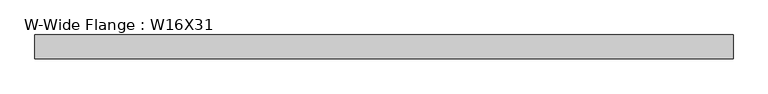
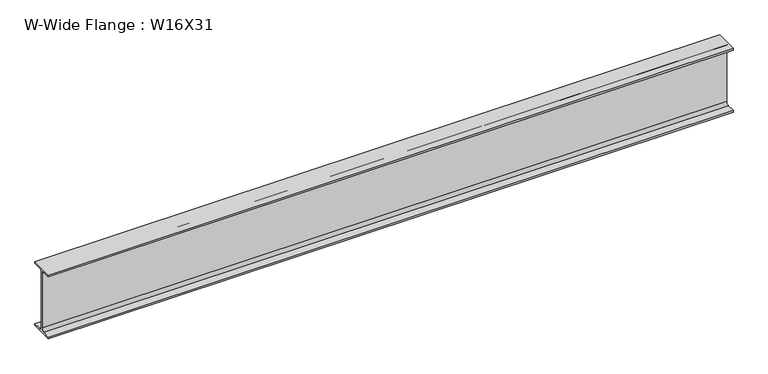
"""IFC4 building model written with IfcOpenShell, lengths in millimetres: beam geometry, W-Wide Flange : W16X31."""

from ifc_helpers import new_model, si_unit, point, frame, frame_2d, origin, place, context, project, spatial, polyline, circle_curve, trimmed, segment, composite_curve, outline, extrude, source, transform, mapped, element, save


def w_wide_flange_w16x31_034e3d4c(model_context):
    return source(origin(), model_context, "Body", "SweptSolid", [
        extrude(outline(composite_curve([segment(polyline([(70.231, -190.754), (70.231, -201.93), (-70.231, -201.93), (-70.231, -190.754), (-20.8915, -190.754)]), True, "CONTINUOUS"), segment(trimmed(circle_curve(frame_2d((-20.8915, -173.355)), 17.399), [point((-20.8915, -190.754))], [point((-3.4925, -173.355))], True, "CARTESIAN"), True, "CONTINUOUS"), segment(polyline([(-3.4925, -173.355), (-3.4925, 173.355)]), True, "CONTINUOUS"), segment(trimmed(circle_curve(frame_2d((-20.8915, 173.355)), 17.399), [point((-3.4925, 173.355))], [point((-20.8915, 190.754))], True, "CARTESIAN"), True, "CONTINUOUS"), segment(polyline([(-20.8915, 190.754), (-70.231, 190.754), (-70.231, 201.93), (70.231, 201.93), (70.231, 190.754), (20.8915, 190.754)]), True, "CONTINUOUS"), segment(trimmed(circle_curve(frame_2d((20.8915, 173.355)), 17.399), [point((20.8915, 190.754))], [point((3.4925, 173.355))], True, "CARTESIAN"), True, "CONTINUOUS"), segment(polyline([(3.4925, 173.355), (3.4925, -173.355)]), True, "CONTINUOUS"), segment(trimmed(circle_curve(frame_2d((20.8915, -173.355)), 17.399), [point((3.4925, -173.355))], [point((20.8915, -190.754))], True, "CARTESIAN"), True, "CONTINUOUS"), segment(polyline([(20.8915, -190.754), (70.231, -190.754)]), True, "CONTINUOUS")], self_intersect=False)), frame((-2052.124346, 0.0, 0.0), z_axis=(1.0, 0.0, 0.0), x_axis=(0.0, 1.0, 0.0)), (0.0, 0.0, 1.0), 4104.248692),
    ])


if __name__ == "__main__":
    model = new_model("IFC4")
    model_context = context("Model", 3, world=origin())
    ifc_project = project(units=[si_unit("LENGTHUNIT", "METRE", prefix="MILLI")], contexts=[model_context])
    site = spatial("IfcSite", under=ifc_project)
    building = spatial("IfcBuilding", under=site)
    placement = place(None, origin())
    w_wide_flange_w16x31_shape = w_wide_flange_w16x31_034e3d4c(model_context)
    element("IfcBeam", 1, ObjectType="W-Wide Flange : W16X31", at=placement, inside=building, context=model_context, shape_type="MappedRepresentation", body=[
        mapped(w_wide_flange_w16x31_shape, transform((0.0, 0.0, 0.0), x_axis=(1.0, 0.0, 0.0), y_axis=(0.0, 1.0, 0.0), z_axis=(0.0, 0.0, 1.0))),
    ])
    save(model, "model.ifc")

# Revit data of these elements
# Type "W-Wide Flange : W16X31"
#   Assembly Code = "B10"
#   W = 31
#   Start Extension Calculation [instance default] = 10' - 0"
#   Start Extension [instance default] = -0' - 0 1/2"
#   End Extension Calculation [instance default] = 10' - 0"
#   End Extension [instance default] = -0' - 0 1/2"
#   Length [instance default] = 5' - 0"
#   bf = 0' - 5.53"
#   d = 1' - 3.9"
#   k = 0' - 1 1/8"
#   k2 = 0' - 0.685"
#   tf = 0' - 0.44"
#   tw = 0' - 0.275"
#   A = 0.0634028 SF
#   Beam Material [instance default] = Metal - Steel - ASTM A992
# Element 1 (IfcBeam, "W-Wide Flange : W16X31")
#   Materials on its faces: "Metal - Steel - ASTM A992"
# Materials
#   "Metal - Steel - ASTM A992": class "Metal", colour RGB 128 0 0, transparency 0
